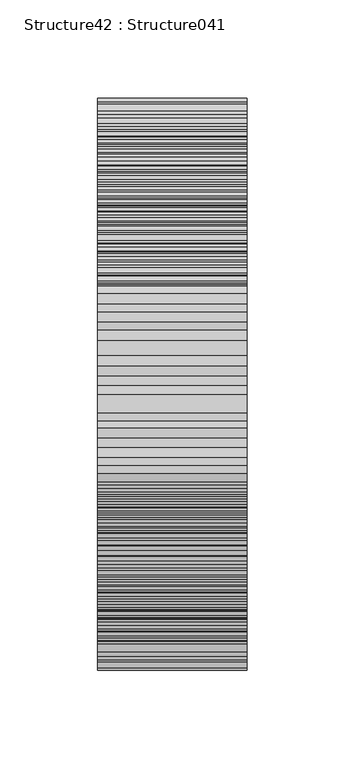
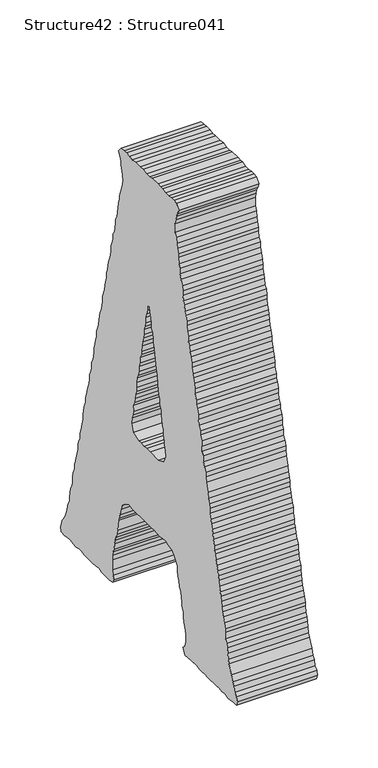
"""IFC4 building model written with IfcOpenShell, lengths in millimetres: proxy geometry, Structure42 : Structure041."""

from ifc_helpers import new_model, si_unit, frame, origin, place, context, project, spatial, polyline, outline, extrude, source, transform, mapped, element, save


def structure42_structure041_00525c18(model_context):
    return source(origin(), model_context, "Body", "SweptSolid", [
        extrude(outline(polyline([(256487.3163609, 3818.8310229), (256489.6558742, 3824.1149855), (256490.2576009, 3828.2163546), (256490.8368631, 3833.4730389), (256492.5762544, 3838.1761347), (256493.1779811, 3841.6741725), (256494.9382322, 3846.9757858), (256494.9382322, 3851.6612309), (256496.6984834, 3856.9179152), (256497.8570078, 3861.0192843), (256499.0379967, 3866.3032469), (256500.1981258, 3870.4030114), (256500.777388, 3875.0772243), (256502.5376391, 3878.5784713), (256503.1393658, 3884.4609514), (256503.1393658, 3888.5623205), (256504.3203547, 3893.822214), (256506.0806058, 3896.763454), (256507.2182704, 3902.6314927), (256508.3992593, 3906.1487857), (256509.5802482, 3910.8310217), (256509.5802482, 3915.5068392), (256510.7612372, 3919.6066036), (256512.5214883, 3924.8905662), (256514.259275, 3929.5904528), (256514.259275, 3934.8503464), (256516.0211307, 3938.3499888), (256517.2021196, 3944.235678), (256517.2021196, 3947.7337158), (256518.9623707, 3952.435207), (256519.541633, 3957.1190475), (256520.7226219, 3962.3757319), (256522.4620131, 3966.5043792), (256522.4620131, 3974.7055128), (256521.3018841, 3979.3781211), (256520.1208952, 3984.0635662), (256518.360644, 3987.5792547), (256516.0211307, 3992.2614906), (256520.1208952, 3996.9645864), (256524.2222643, 3997.5486624), (256528.3444932, 3997.5486624), (256533.6043868, 3996.390138), (256538.2850181, 3996.390138), (256543.5657715, 3997.5486624), (256547.0654139, 3996.9645864), (256551.1876428, 3997.5486624), (256560.5489054, 3997.5486624), (256565.2503966, 3996.390138), (256569.9310279, 3996.390138), (256575.1909215, 3997.5486624), (256580.4941393, 3996.9645864), (256588.0935462, 3996.9645864), (256593.3759042, 3996.390138), (256597.4548088, 3997.5486624), (256602.7580267, 3997.5486624), (256606.8369313, 3996.9645864), (256612.0968249, 3996.390138), (256615.6397916, 3991.6806238), (256613.2778138, 3987.5792547), (256612.0968249, 3983.4794902), (256611.5384225, 3979.9621971), (256610.3574336, 3974.7055128), (256608.5971825, 3965.8930249), (256609.7781714, 3961.794865), (256610.9591603, 3956.5349715), (256614.4588027, 3947.1496398), (256614.4588027, 3944.235678), (256615.6397916, 3938.9517154), (256616.798316, 3934.2758979), (256617.4000427, 3928.9919353), (256618.5585672, 3924.2888396), (256620.8996851, 3919.6066036), (256620.8996851, 3916.0909152), (256621.4789474, 3910.8310217), (256622.6599363, 3906.1487857), (256625.0219141, 3902.6314927), (256625.0219141, 3897.3475301), (256626.7613054, 3892.6636896), (256627.9198298, 3888.5623205), (256627.9198298, 3883.8881076), (256629.1008187, 3878.5784713), (256630.8610698, 3873.9203044), (256632.621321, 3869.8189354), (256633.2230477, 3866.3032469), (256633.8023099, 3861.0192843), (256635.5417012, 3856.9179152), (256635.5417012, 3851.6612309), (256637.3019523, 3846.9757858), (256637.903679, 3842.8583706), (256639.0622034, 3837.6000817), (256641.9825836, 3829.374879), (256641.9825836, 3824.1149855), (256643.1635725, 3820.015221), (256644.3445614, 3815.3313805), (256646.6840748, 3810.0474179), (256647.2858015, 3806.5317294), (256648.4443259, 3801.8462843), (256649.0460526, 3797.1463977), (256650.7854439, 3791.8865042), (256651.9664328, 3788.3611881), (256651.9664328, 3783.0868532), (256653.7266839, 3777.8285642), (256654.3059461, 3774.3032481), (256656.0661973, 3769.0176809), (256656.6470641, 3764.3611187), (256657.2263263, 3759.6596275), (256658.4073152, 3756.1423345), (256660.1675663, 3751.4424479), (256660.7468286, 3745.6000829), (256661.9278175, 3740.9162424), (256663.6880686, 3737.9750024), (256663.6880686, 3732.7167134), (256664.8481977, 3727.4311462), (256666.6084488, 3723.3313817), (256667.7669732, 3718.0554422), (256668.9479621, 3714.5301261), (256670.1289511, 3710.4560353), (256670.1289511, 3705.7545441), (256672.4476046, 3699.8881101), (256673.6285935, 3695.2122926), (256674.2303201, 3691.0868544), (256674.2303201, 3686.4030139), (256675.3888446, 3682.8857208), (256677.1490957, 3677.0449605), (256677.7508224, 3673.5276674), (256679.4902137, 3668.8261762), (256679.4902137, 3663.5598643), (256681.829727, 3659.4584952), (256683.0107159, 3655.3587307), (256683.0107159, 3650.6845178), (256684.1917049, 3645.4262289), (256685.951956, 3640.114988), (256687.112085, 3636.0408972), (256688.2706095, 3632.5155811), (256688.8723362, 3627.2396415), (256690.6325873, 3622.555801), (256691.8135762, 3617.2718384), (256691.8135762, 3612.5976255), (256692.3928384, 3608.4705827), (256694.7114919, 3604.3964919), (256695.8924808, 3599.1125293), (256697.0734697, 3594.4286888), (256697.0734697, 3590.3289243), (256698.8337209, 3586.2115092), (256701.7541011, 3576.2693797), (256703.5143522, 3572.1423369), (256705.2746033, 3568.6426945), (256708.7967102, 3563.366755), (256709.9552346, 3560.441561), (256711.7154858, 3555.1848766), (256710.5344969, 3551.0658569), (256704.6953411, 3550.4833855), (256701.1956987, 3551.0658569), (256695.8924808, 3551.6675836), (256691.2118495, 3550.4833855), (256685.951956, 3550.4833855), (256681.2504648, 3551.6675836), (256677.1490957, 3551.6675836), (256672.4476046, 3551.0658569), (256668.3686999, 3551.0658569), (256662.5070797, 3550.4833855), (256658.4073152, 3550.4833855), (256653.7266839, 3551.0658569), (256648.4443259, 3551.6675836), (256644.3445614, 3550.4833855), (256630.8610698, 3550.4833855), (256625.6011763, 3551.6675836), (256623.2391985, 3555.7416744), (256625.0219141, 3559.2669905), (256626.1804385, 3563.9412034), (256626.1804385, 3573.9266571), (256626.1804385, 3578.6104977), (256625.0219141, 3582.7102621), (256623.2391985, 3586.2115092), (256622.6599363, 3592.0955938), (256621.4789474, 3596.1953583), (256619.7186962, 3600.2967274), (256618.5585672, 3604.3964919), (256617.4000427, 3609.0723094), (256616.2190538, 3619.6145609), (256615.0380649, 3622.555801), (256613.2778138, 3627.2396415), (256612.0968249, 3633.0980525), (256609.1989091, 3638.9580681), (256605.0766802, 3642.4833842), (256598.6357978, 3645.9830266), (256593.9551664, 3644.8245022), (256584.573044, 3644.8245022), (256578.7114237, 3645.4262289), (256566.4313855, 3645.4262289), (256561.1281677, 3644.8245022), (256557.049263, 3645.9830266), (256552.3477719, 3645.4262289), (256547.6671406, 3644.8245022), (256543.5657715, 3645.4262289), (256537.7057558, 3645.9830266), (256534.183649, 3644.8245022), (256527.1635043, 3643.0578326), (256523.643002, 3639.5405396), (256518.9623707, 3633.0980525), (256518.9623707, 3627.8397636), (256517.7813818, 3622.555801), (256516.0211307, 3619.6145609), (256515.4418685, 3613.772196), (256513.1007505, 3610.2292293), (256511.9197616, 3604.9709403), (256511.3404994, 3601.4536473), (256511.3404994, 3596.7698067), (256508.9785216, 3592.0955938), (256508.3992593, 3587.3860796), (256507.8199971, 3582.7102621), (256506.0806058, 3578.6104977), (256504.3203547, 3572.7440636), (256504.8996169, 3565.1254015), (256506.6598681, 3559.2669905), (256509.5802482, 3556.3417965), (256506.0806058, 3550.4833855), (256500.777388, 3551.0658569), (256496.0967567, 3551.6675836), (256486.7146342, 3551.6675836), (256482.0564673, 3551.0658569), (256477.3533716, 3551.0658569), (256473.2536071, 3551.6675836), (256469.1297735, 3551.0658569), (256463.2922224, 3551.0658569), (256459.7701155, 3551.6675836), (256453.9309597, 3551.0658569), (256450.4104575, 3551.6675836), (256445.7298262, 3550.4833855), (256440.4266083, 3551.6675836), (256435.1667148, 3550.4833855), (256431.0653457, 3551.0658569), (256426.3638545, 3551.6675836), (256421.7056876, 3551.6675836), (256419.922972, 3556.3417965), (256421.103961, 3560.441561), (256424.045201, 3563.366755), (256425.2037254, 3568.6426945), (256426.9655812, 3572.1423369), (256429.3050945, 3577.4535778), (256433.4064636, 3586.2115092), (256434.5874525, 3589.7544759), (256435.1667148, 3595.5872132), (256436.3477037, 3600.2967274), (256437.5062281, 3604.3964919), (256439.2664792, 3607.8961343), (256439.8457415, 3613.772196), (256439.8457415, 3617.2718384), (256441.028335, 3622.555801), (256442.7885861, 3627.8397636), (256444.5488372, 3631.915459), (256445.7298262, 3636.0408972), (256446.3090884, 3641.2991861), (256446.8658861, 3645.9830266), (256447.4676128, 3650.1004418), (256449.8087308, 3654.1841602), (256450.4104575, 3660.0682449), (256450.9897197, 3664.1423357), (256451.5689819, 3668.8261762), (256453.329233, 3672.9435914), (256455.0894842, 3677.6274319), (256456.2496132, 3682.8857208), (256457.4306021, 3685.8285655), (256457.4306021, 3690.512406), (256459.1908533, 3695.786741), (256459.7701155, 3701.0723082), (256460.9511044, 3704.5879966), (256462.6904957, 3709.2718371), (256463.2922224, 3713.3555556), (256465.0524735, 3718.6571688), (256465.0524735, 3723.3313817), (256466.2334624, 3727.4311462), (256467.3919868, 3732.1149867), (256468.5729758, 3737.400554), (256470.9140937, 3746.1745313), (256472.0726182, 3750.8583719), (256472.0726182, 3755.559863), (256473.8328693, 3759.6596275), (256475.5931204, 3763.759392), (256475.5931204, 3769.6274306), (256477.9342384, 3773.11905), (256477.9342384, 3777.8285642), (256478.5135006, 3783.0868532), (256480.8754784, 3787.7867397), (256480.8754784, 3791.8865042), (256483.2149918, 3795.960595), (256483.8167185, 3801.8462843), (256483.8167185, 3805.9476534), (256486.135372, 3811.2043377), (256487.3163609, 3814.7296538), (256487.3163609, 3818.8310229)]), holes=[polyline([(256550.0066539, 3720.4158154), (256563.4901455, 3720.4158154), (256568.750039, 3720.9726131), (256574.0307924, 3719.8140887), (256578.1321615, 3720.9726131), (256582.2335306, 3720.4158154), (256591.0139264, 3723.3313817), (256593.9551664, 3730.9323932), (256592.7741775, 3736.7988273), (256591.6156531, 3740.9162424), (256590.4346642, 3744.9999608), (256591.0139264, 3750.8583719), (256588.6952729, 3754.9854146), (256588.0935462, 3759.6596275), (256587.514284, 3763.759392), (256585.7540329, 3767.8607611), (256585.1523062, 3772.5606477), (256585.1523062, 3777.2444882), (256584.573044, 3782.5027771), (256582.8127928, 3786.0280932), (256581.6526638, 3790.7039107), (256581.6526638, 3795.4037973), (256579.3131504, 3800.6717138), (256579.3131504, 3805.9476534), (256577.5528993, 3810.0474179), (256576.9511726, 3813.5743386), (256576.3719104, 3819.4150989), (256575.1909215, 3824.1149855), (256574.0307924, 3828.790803), (256573.4515302, 3832.8921721), (256573.4515302, 3837.6000817), (256571.1120168, 3842.2758992), (256570.5102902, 3846.3772683), (256570.5102902, 3851.6612309), (256568.750039, 3856.3161885), (256567.5690501, 3860.4432313), (256567.5690501, 3864.5446004), (256565.8296588, 3865.1190488), (256564.6711344, 3860.4432313), (256562.8884188, 3855.7353217), (256562.3091566, 3851.0595042), (256562.3091566, 3845.8012153), (256559.9696432, 3842.2758992), (256559.3679165, 3836.9919366), (256559.3679165, 3833.4730389), (256557.049263, 3828.790803), (256556.4475364, 3822.932392), (256555.8682741, 3818.8310229), (256554.6872852, 3814.7296538), (256554.108023, 3810.0474179), (256552.3477719, 3804.7730829), (256551.7460452, 3795.4037973), (256550.6083806, 3790.7039107), (256550.0066539, 3786.0280932), (256548.2464028, 3783.0868532), (256548.2464028, 3777.8285642), (256545.9068894, 3773.11905), (256545.9068894, 3768.4432325), (256544.7259005, 3764.3611187), (256544.1450337, 3759.0595054), (256542.407247, 3755.559863), (256542.407247, 3750.3015741), (256540.6245314, 3744.9999608), (256540.6245314, 3741.5003184), (256539.466007, 3736.7988273), (256538.2850181, 3730.9323932), (256541.8055203, 3723.9154578), (256550.0066539, 3720.4158154)])]), frame((-38594.2176606, 0.0, 0.0), z_axis=(1.0, 0.0, 0.0), x_axis=(0.0, 1.0, 0.0)), (0.0, 0.0, 1.0), 76.2),
    ])


if __name__ == "__main__":
    model = new_model("IFC4")
    model_context = context("Model", 3, world=origin())
    ifc_project = project(units=[si_unit("LENGTHUNIT", "METRE", prefix="MILLI")], contexts=[model_context])
    site = spatial("IfcSite", under=ifc_project)
    building = spatial("IfcBuilding", under=site)
    placement = place(None, origin())
    structure42_structure041_shape = structure42_structure041_00525c18(model_context)
    element("IfcBuildingElementProxy", 1, Name="Structure42 : Structure041", ObjectType="Structure42 : Structure041", at=placement, inside=building, context=model_context, shape_type="MappedRepresentation", body=[
        mapped(structure42_structure041_shape, transform((0.0, 0.0, 0.0), x_axis=(1.0, 0.0, 0.0), y_axis=(0.0, 1.0, 0.0), z_axis=(0.0, 0.0, 1.0))),
    ])
    save(model, "model.ifc")

# Revit data of these elements
# Project information
#   Project Issue Date = "06/14/2019"
#   Project Status = "Project Status"
#   Client Name = "Owner"
#   Project Address = "SOMERS, WI"
#   Project Name = "OAKFIRE 2.0"
#   Project Number = "Project Number"
# Type "Structure42 : Structure041"
#   NameOverride = "Structure041"
# Element 1 (IfcBuildingElementProxy, "Structure42 : Structure041")
#   Materials on its faces: "BRUSHED ALUM. LETTERING"
# Materials
#   "BRUSHED ALUM. LETTERING": class "Unassigned", colour RGB 169 181 186, transparency 0, Cost = 0
